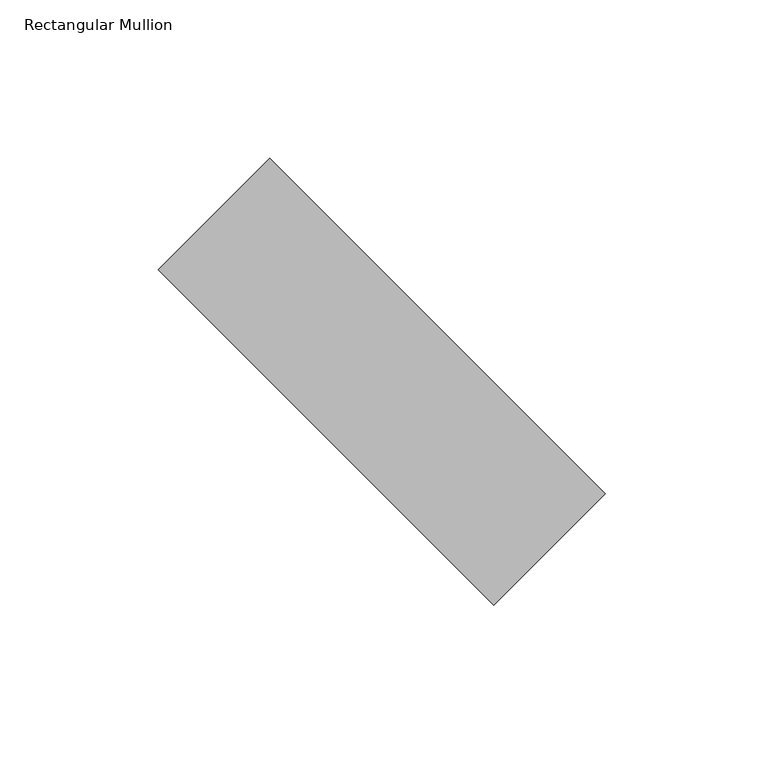
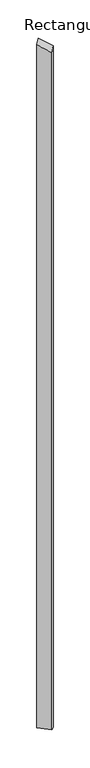
"""IFC4 building model written with IfcOpenShell, lengths in millimetres: member geometry, Rectangular Mullion : tilted mullions."""

from ifc_helpers import new_model, si_unit, origin, place, context, project, spatial, faceted_brep, source, transform, mapped, element, save


def rectangular_mullion_b81ce2a0(model_context):
    return source(origin(), model_context, "Body", "Brep", [
        faceted_brep([(-35.3553391, 70.7106781, -7999.1836632), (70.7106781, -35.3553391, -7999.1836632), (35.3553391, -70.7106781, -7999.1836632), (-70.7106781, 35.3553391, -7999.1836632), (-70.7106781, 35.3553391, 10.0709562), (-35.3553391, 70.7106781, 55.104478), (35.3553391, -70.7106781, -55.104478), (70.7106781, -35.3553391, -10.0709562)], [[[0, 1, 2, 3]], [[4, 5, 0, 3]], [[6, 4, 3, 2]], [[7, 6, 2, 1]], [[5, 7, 1, 0]], [[5, 4, 6, 7]]]),
    ])


if __name__ == "__main__":
    model = new_model("IFC4")
    model_context = context("Model", 3, world=origin())
    ifc_project = project(units=[si_unit("LENGTHUNIT", "METRE", prefix="MILLI")], contexts=[model_context])
    site = spatial("IfcSite", under=ifc_project)
    building = spatial("IfcBuilding", under=site)
    placement = place(None, origin())
    rectangular_mullion_shape = rectangular_mullion_b81ce2a0(model_context)
    element("IfcMember", 1, ObjectType="Rectangular Mullion : tilted mullions", at=placement, inside=building, context=model_context, shape_type="MappedRepresentation", body=[
        mapped(rectangular_mullion_shape, transform((0.0, 0.0, 0.0), x_axis=(1.0, 0.0, 0.0), y_axis=(0.0, 1.0, 0.0), z_axis=(0.0, 0.0, 1.0))),
    ])
    save(model, "model.ifc")

# Revit data of these elements
# Type "Rectangular Mullion : tilted mullions"
#   built-in parameter 1007304 = 0.492126 (stored number, unit not read)
#   built-in parameter 1007301 = 0.082021 (stored number, unit not read)
#   built-in parameter 1007300 = 0.082021 (stored number, unit not read)
# Element 1 (IfcMember, "Rectangular Mullion : tilted mullions")
#   Materials on its faces: "Aluminum"
# Materials
#   "Aluminum": class "Metal", colour RGB 244 244 244, transparency 0, Description = "Aluminum 6061", Cost = 0
